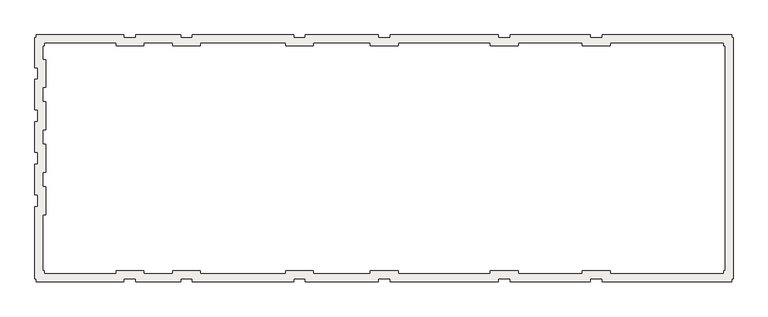
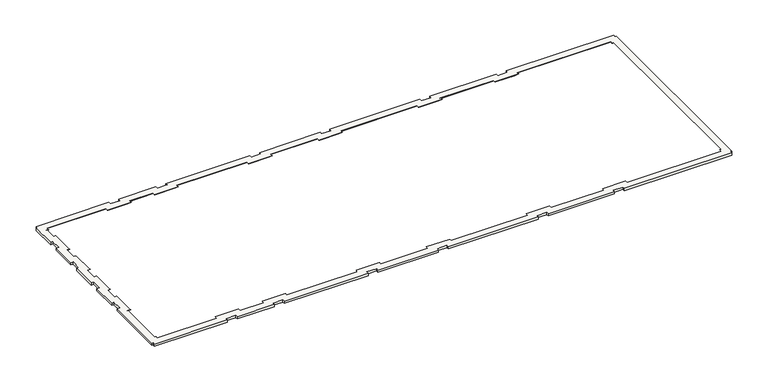
"""IFC4 building model written with IfcOpenShell, lengths in millimetres: slab geometry, HAUNCH FOR SOG : FTS801_Haunch_GS."""

from ifc_helpers import new_model, si_unit, origin, place, context, project, spatial, faceted_brep, source, transform, mapped, element, save


def slab_ae3d626d(model_context):
    return source(origin(), model_context, "Body", "Brep", [
        faceted_brep([(370.0, 38729.5208589, 399.9720055), (370.0, 38729.5208589, 199.9720055), (370.0, 38529.5208589, 199.9720055), (370.0, 38529.5208589, 399.9720055), (770.0, 38329.5208589, 199.9720055), (970.0, 38129.5208589, 399.9720055), (970.0, 37929.5208589, 399.9720055), (770.0, 38129.5208589, 199.9720055), (270.0, 38529.5208589, 199.9720055), (270.0, 38529.5208589, 399.9720055), (870.0, 37929.5208589, 399.9720055), (670.0, 38129.5208589, 199.9720055), (270.0, 36419.5208589, 199.9720055), (270.0, 36419.5208589, 399.9720055), (870.0, 37019.5208589, 399.9720055), (670.0, 36819.5208589, 199.9720055), (470.0, 36419.5208589, 199.9720055), (470.0, 36419.5208589, 399.9720055), (405.0, 36419.5208589, 399.9720055), (1070.0, 37019.5208589, 399.9720055), (870.0, 36819.5208589, 199.9720055), (470.0, 35579.5208589, 199.9720055), (470.0, 35579.5208589, 399.9720055), (1070.0, 34979.5208589, 399.9720055), (870.0, 35179.5208589, 199.9720055), (270.0, 35579.5208589, 199.9720055), (270.0, 35579.5208589, 399.9720055), (405.0, 35579.5208589, 399.9720055), (870.0, 34979.5208589, 399.9720055), (670.0, 35179.5208589, 199.9720055), (270.0, 33419.5208589, 199.9720055), (270.0, 33419.5208589, 399.9720055), (870.0, 34019.5208589, 399.9720055), (670.0, 33819.5208589, 199.9720055), (470.0, 33419.5208589, 199.9720055), (470.0, 33419.5208589, 399.9720055), (405.0, 33419.5208589, 399.9720055), (1070.0, 34019.5208589, 399.9720055), (870.0, 33819.5208589, 199.9720055), (470.0, 32579.5208589, 199.9720055), (470.0, 32579.5208589, 399.9720055), (1070.0, 31979.5208589, 399.9720055), (870.0, 32179.5208589, 199.9720055), (270.0, 32579.5208589, 199.9720055), (270.0, 32579.5208589, 399.9720055), (405.0, 32579.5208589, 399.9720055), (870.0, 31979.5208589, 399.9720055), (670.0, 32179.5208589, 199.9720055), (270.0, 30419.5208589, 199.9720055), (270.0, 30419.5208589, 399.9720055), (870.0, 31019.5208589, 399.9720055), (670.0, 30819.5208589, 199.9720055), (470.0, 30419.5208589, 199.9720055), (470.0, 30419.5208589, 399.9720055), (405.0, 30419.5208589, 399.9720055), (1070.0, 31019.5208589, 399.9720055), (870.0, 30819.5208589, 199.9720055), (470.0, 29579.5208589, 199.9720055), (470.0, 29579.5208589, 399.9720055), (1070.0, 28979.5208589, 399.9720055), (870.0, 29179.5208589, 199.9720055), (270.0, 29579.5208589, 199.9720055), (270.0, 29579.5208589, 399.9720055), (405.0, 29579.5208589, 399.9720055), (870.0, 28979.5208589, 399.9720055), (670.0, 29179.5208589, 199.9720055), (270.0, 27419.5208589, 199.9720055), (270.0, 27419.5208589, 399.9720055), (870.0, 28019.5208589, 399.9720055), (670.0, 27819.5208589, 199.9720055), (470.0, 27419.5208589, 199.9720055), (470.0, 27419.5208589, 399.9720055), (405.0, 27419.5208589, 399.9720055), (1070.0, 28019.5208589, 399.9720055), (870.0, 27819.5208589, 199.9720055), (470.0, 26579.5208589, 199.9720055), (470.0, 26579.5208589, 399.9720055), (1070.0, 25979.5208589, 399.9720055), (870.0, 26179.5208589, 199.9720055), (270.0, 26579.5208589, 199.9720055), (270.0, 26579.5208589, 399.9720055), (405.0, 26579.5208589, 399.9720055), (870.0, 25979.5208589, 399.9720055), (670.0, 26179.5208589, 199.9720055), (270.0, 21469.5208589, 199.9720055), (270.0, 21469.5208589, 399.9720055), (870.0, 22069.5208589, 399.9720055), (670.0, 21869.5208589, 199.9720055), (370.0, 21469.5208589, 199.9720055), (370.0, 21469.5208589, 399.9720055), (970.0, 22069.5208589, 399.9720055), (770.0, 21869.5208589, 199.9720055), (370.0, 21269.5208589, 199.9720055), (370.0, 21269.5208589, 399.9720055), (970.0, 21869.5208589, 399.9720055), (770.0, 21669.5208589, 199.9720055), (6574.0, 21269.5208589, 199.9720055), (6574.0, 21269.5208589, 399.9720055), (5974.0, 21869.5208589, 399.9720055), (6174.0, 21669.5208589, 199.9720055), (6574.0, 21469.5208589, 199.9720055), (6574.0, 21469.5208589, 399.9720055), (5974.0, 22069.5208589, 399.9720055), (6174.0, 21869.5208589, 199.9720055), (7414.0, 21469.5208589, 199.9720055), (7414.0, 21469.5208589, 399.9720055), (8014.0, 22069.5208589, 399.9720055), (7814.0, 21869.5208589, 199.9720055), (7414.0, 21269.5208589, 199.9720055), (7414.0, 21269.5208589, 399.9720055), (8014.0, 21869.5208589, 399.9720055), (7814.0, 21669.5208589, 199.9720055), (10574.0, 21269.5208589, 199.9720055), (10574.0, 21269.5208589, 399.9720055), (9974.0, 21869.5208589, 399.9720055), (10174.0, 21669.5208589, 199.9720055), (10574.0, 21469.5208589, 199.9720055), (10574.0, 21469.5208589, 399.9720055), (9974.0, 22069.5208589, 399.9720055), (10174.0, 21869.5208589, 199.9720055), (11414.0, 21469.5208589, 199.9720055), (11414.0, 21469.5208589, 399.9720055), (12014.0, 22069.5208589, 399.9720055), (11814.0, 21869.5208589, 199.9720055), (11414.0, 21269.5208589, 199.9720055), (11414.0, 21269.5208589, 399.9720055), (12014.0, 21869.5208589, 399.9720055), (11814.0, 21669.5208589, 199.9720055), (18574.0, 21269.5208589, 199.9720055), (18574.0, 21269.5208589, 399.9720055), (17974.0, 21869.5208589, 399.9720055), (18174.0, 21669.5208589, 199.9720055), (18574.0, 21469.5208589, 199.9720055), (18574.0, 21469.5208589, 399.9720055), (17974.0, 22069.5208589, 399.9720055), (18174.0, 21869.5208589, 199.9720055), (19414.0, 21469.5208589, 199.9720055), (19414.0, 21469.5208589, 399.9720055), (20014.0, 22069.5208589, 399.9720055), (19814.0, 21869.5208589, 199.9720055), (19414.0, 21269.5208589, 199.9720055), (19414.0, 21269.5208589, 399.9720055), (20014.0, 21869.5208589, 399.9720055), (19814.0, 21669.5208589, 199.9720055), (24574.0, 21269.5208589, 199.9720055), (24574.0, 21269.5208589, 399.9720055), (23974.0, 21869.5208589, 399.9720055), (24174.0, 21669.5208589, 199.9720055), (24574.0, 21469.5208589, 199.9720055), (24574.0, 21469.5208589, 399.9720055), (23974.0, 22069.5208589, 399.9720055), (24174.0, 21869.5208589, 199.9720055), (25414.0, 21469.5208589, 199.9720055), (25414.0, 21469.5208589, 399.9720055), (26014.0, 22069.5208589, 399.9720055), (25814.0, 21869.5208589, 199.9720055), (25414.0, 21269.5208589, 199.9720055), (25414.0, 21269.5208589, 399.9720055), (26014.0, 21869.5208589, 399.9720055), (25814.0, 21669.5208589, 199.9720055), (33074.0, 21269.5208589, 199.9720055), (33074.0, 21269.5208589, 399.9720055), (32474.0, 21869.5208589, 399.9720055), (32674.0, 21669.5208589, 199.9720055), (33074.0, 21469.5208589, 199.9720055), (33074.0, 21469.5208589, 399.9720055), (32474.0, 22069.5208589, 399.9720055), (32674.0, 21869.5208589, 199.9720055), (33914.0, 21469.5208589, 199.9720055), (33914.0, 21469.5208589, 399.9720055), (34514.0, 22069.5208589, 399.9720055), (34314.0, 21869.5208589, 199.9720055), (33914.0, 21269.5208589, 199.9720055), (33914.0, 21269.5208589, 399.9720055), (34514.0, 21869.5208589, 399.9720055), (34314.0, 21669.5208589, 199.9720055), (39574.0, 21269.5208589, 199.9720055), (39574.0, 21269.5208589, 399.9720055), (38974.0, 21869.5208589, 399.9720055), (39174.0, 21669.5208589, 199.9720055), (39574.0, 21469.5208589, 199.9720055), (39574.0, 21469.5208589, 399.9720055), (38974.0, 22069.5208589, 399.9720055), (39174.0, 21869.5208589, 199.9720055), (40414.0, 21469.5208589, 199.9720055), (40414.0, 21469.5208589, 399.9720055), (41014.0, 22069.5208589, 399.9720055), (40814.0, 21869.5208589, 199.9720055), (40414.0, 21269.5208589, 199.9720055), (40414.0, 21269.5208589, 399.9720055), (41014.0, 21869.5208589, 399.9720055), (40814.0, 21669.5208589, 199.9720055), (49580.0, 21269.5208589, 199.9720055), (49580.0, 21269.5208589, 399.9720055), (48980.0, 21869.5208589, 399.9720055), (49180.0, 21669.5208589, 199.9720055), (49580.0, 21469.5208589, 199.9720055), (49580.0, 21469.5208589, 399.9720055), (48980.0, 22069.5208589, 399.9720055), (49180.0, 21869.5208589, 199.9720055), (49680.0, 21469.5208589, 199.9720055), (49680.0, 21469.5208589, 399.9720055), (49595.0, 21469.5208589, 399.9720055), (49080.0, 22069.5208589, 399.9720055), (49280.0, 21869.5208589, 199.9720055), (49680.0, 38529.5208589, 199.9720055), (49680.0, 38529.5208589, 399.9720055), (49080.0, 37929.5208589, 399.9720055), (49280.0, 38129.5208589, 199.9720055), (49580.0, 38529.5208589, 199.9720055), (49580.0, 38529.5208589, 399.9720055), (49595.0, 38529.5208589, 399.9720055), (48980.0, 37929.5208589, 399.9720055), (49180.0, 38129.5208589, 199.9720055), (49580.0, 38729.5208589, 199.9720055), (49580.0, 38729.5208589, 399.9720055), (48980.0, 38129.5208589, 399.9720055), (49180.0, 38329.5208589, 199.9720055), (40414.0, 38729.5208589, 199.9720055), (40414.0, 38729.5208589, 399.9720055), (41014.0, 38129.5208589, 399.9720055), (40814.0, 38329.5208589, 199.9720055), (40414.0, 38529.5208589, 199.9720055), (40414.0, 38529.5208589, 399.9720055), (41014.0, 37929.5208589, 399.9720055), (40814.0, 38129.5208589, 199.9720055), (39574.0, 38529.5208589, 199.9720055), (39574.0, 38529.5208589, 399.9720055), (38974.0, 37929.5208589, 399.9720055), (39174.0, 38129.5208589, 199.9720055), (39574.0, 38729.5208589, 199.9720055), (39574.0, 38729.5208589, 399.9720055), (38974.0, 38129.5208589, 399.9720055), (39174.0, 38329.5208589, 199.9720055), (33914.0, 38729.5208589, 199.9720055), (33914.0, 38729.5208589, 399.9720055), (34514.0, 38129.5208589, 399.9720055), (34314.0, 38329.5208589, 199.9720055), (33914.0, 38529.5208589, 199.9720055), (33914.0, 38529.5208589, 399.9720055), (34514.0, 37929.5208589, 399.9720055), (34314.0, 38129.5208589, 199.9720055), (33074.0, 38529.5208589, 199.9720055), (33074.0, 38529.5208589, 399.9720055), (32474.0, 37929.5208589, 399.9720055), (32674.0, 38129.5208589, 199.9720055), (33074.0, 38729.5208589, 199.9720055), (33074.0, 38729.5208589, 399.9720055), (32474.0, 38129.5208589, 399.9720055), (32674.0, 38329.5208589, 199.9720055), (25414.0, 38729.5208589, 199.9720055), (25414.0, 38729.5208589, 399.9720055), (26014.0, 38129.5208589, 399.9720055), (25814.0, 38329.5208589, 199.9720055), (25414.0, 38529.5208589, 199.9720055), (25414.0, 38529.5208589, 399.9720055), (26014.0, 37929.5208589, 399.9720055), (25814.0, 38129.5208589, 199.9720055), (24574.0, 38529.5208589, 199.9720055), (24574.0, 38529.5208589, 399.9720055), (23974.0, 37929.5208589, 399.9720055), (24174.0, 38129.5208589, 199.9720055), (24574.0, 38729.5208589, 199.9720055), (24574.0, 38729.5208589, 399.9720055), (23974.0, 38129.5208589, 399.9720055), (24174.0, 38329.5208589, 199.9720055), (19414.0, 38729.5208589, 199.9720055), (19414.0, 38729.5208589, 399.9720055), (20014.0, 38129.5208589, 399.9720055), (19814.0, 38329.5208589, 199.9720055), (19414.0, 38529.5208589, 199.9720055), (19414.0, 38529.5208589, 399.9720055), (20014.0, 37929.5208589, 399.9720055), (19814.0, 38129.5208589, 199.9720055), (18574.0, 38529.5208589, 199.9720055), (18574.0, 38529.5208589, 399.9720055), (17974.0, 37929.5208589, 399.9720055), (18174.0, 38129.5208589, 199.9720055), (18574.0, 38729.5208589, 199.9720055), (18574.0, 38729.5208589, 399.9720055), (17974.0, 38129.5208589, 399.9720055), (18174.0, 38329.5208589, 199.9720055), (11414.0, 38729.5208589, 199.9720055), (11414.0, 38729.5208589, 399.9720055), (12014.0, 38129.5208589, 399.9720055), (11814.0, 38329.5208589, 199.9720055), (11414.0, 38529.5208589, 199.9720055), (11414.0, 38529.5208589, 399.9720055), (12014.0, 37929.5208589, 399.9720055), (11814.0, 38129.5208589, 199.9720055), (10574.0, 38529.5208589, 199.9720055), (10574.0, 38529.5208589, 399.9720055), (9974.0, 37929.5208589, 399.9720055), (10174.0, 38129.5208589, 199.9720055), (10574.0, 38729.5208589, 199.9720055), (10574.0, 38729.5208589, 399.9720055), (9974.0, 38129.5208589, 399.9720055), (10174.0, 38329.5208589, 199.9720055), (7414.0, 38729.5208589, 199.9720055), (7414.0, 38729.5208589, 399.9720055), (8014.0, 38129.5208589, 399.9720055), (7814.0, 38329.5208589, 199.9720055), (7414.0, 38529.5208589, 199.9720055), (7414.0, 38529.5208589, 399.9720055), (8014.0, 37929.5208589, 399.9720055), (7814.0, 38129.5208589, 199.9720055), (6574.0, 38529.5208589, 199.9720055), (6574.0, 38529.5208589, 399.9720055), (5974.0, 37929.5208589, 399.9720055), (6174.0, 38129.5208589, 199.9720055), (6574.0, 38729.5208589, 199.9720055), (6574.0, 38729.5208589, 399.9720055), (5974.0, 38129.5208589, 399.9720055), (6174.0, 38329.5208589, 199.9720055)], [[[0, 1, 2, 3]], [[4, 5, 6, 7]], [[3, 2, 8, 9]], [[7, 6, 10, 11]], [[9, 8, 12, 13]], [[11, 10, 14, 15]], [[13, 12, 16, 17, 18]], [[15, 14, 19, 20]], [[17, 16, 21, 22]], [[20, 19, 23, 24]], [[22, 21, 25, 26, 27]], [[24, 23, 28, 29]], [[26, 25, 30, 31]], [[29, 28, 32, 33]], [[31, 30, 34, 35, 36]], [[33, 32, 37, 38]], [[35, 34, 39, 40]], [[38, 37, 41, 42]], [[40, 39, 43, 44, 45]], [[42, 41, 46, 47]], [[44, 43, 48, 49]], [[47, 46, 50, 51]], [[49, 48, 52, 53, 54]], [[51, 50, 55, 56]], [[53, 52, 57, 58]], [[56, 55, 59, 60]], [[58, 57, 61, 62, 63]], [[60, 59, 64, 65]], [[62, 61, 66, 67]], [[65, 64, 68, 69]], [[67, 66, 70, 71, 72]], [[69, 68, 73, 74]], [[71, 70, 75, 76]], [[74, 73, 77, 78]], [[76, 75, 79, 80, 81]], [[78, 77, 82, 83]], [[80, 79, 84, 85]], [[83, 82, 86, 87]], [[85, 84, 88, 89]], [[87, 86, 90, 91]], [[89, 88, 92, 93]], [[91, 90, 94, 95]], [[93, 92, 96, 97]], [[95, 94, 98, 99]], [[97, 96, 100, 101]], [[99, 98, 102, 103]], [[101, 100, 104, 105]], [[103, 102, 106, 107]], [[105, 104, 108, 109]], [[107, 106, 110, 111]], [[109, 108, 112, 113]], [[111, 110, 114, 115]], [[113, 112, 116, 117]], [[115, 114, 118, 119]], [[117, 116, 120, 121]], [[119, 118, 122, 123]], [[121, 120, 124, 125]], [[123, 122, 126, 127]], [[125, 124, 128, 129]], [[127, 126, 130, 131]], [[129, 128, 132, 133]], [[131, 130, 134, 135]], [[133, 132, 136, 137]], [[135, 134, 138, 139]], [[137, 136, 140, 141]], [[139, 138, 142, 143]], [[141, 140, 144, 145]], [[143, 142, 146, 147]], [[145, 144, 148, 149]], [[147, 146, 150, 151]], [[149, 148, 152, 153]], [[151, 150, 154, 155]], [[153, 152, 156, 157]], [[155, 154, 158, 159]], [[157, 156, 160, 161]], [[159, 158, 162, 163]], [[161, 160, 164, 165]], [[163, 162, 166, 167]], [[165, 164, 168, 169]], [[167, 166, 170, 171]], [[169, 168, 172, 173]], [[171, 170, 174, 175]], [[173, 172, 176, 177]], [[175, 174, 178, 179]], [[177, 176, 180, 181]], [[179, 178, 182, 183]], [[181, 180, 184, 185]], [[183, 182, 186, 187]], [[185, 184, 188, 189]], [[187, 186, 190, 191]], [[189, 188, 192, 193]], [[191, 190, 194, 195]], [[193, 192, 196, 197]], [[195, 194, 198, 199]], [[197, 196, 200, 201, 202]], [[199, 198, 203, 204]], [[201, 200, 205, 206]], [[204, 203, 207, 208]], [[206, 205, 209, 210, 211]], [[208, 207, 212, 213]], [[210, 209, 214, 215]], [[213, 212, 216, 217]], [[215, 214, 218, 219]], [[217, 216, 220, 221]], [[219, 218, 222, 223]], [[221, 220, 224, 225]], [[223, 222, 226, 227]], [[225, 224, 228, 229]], [[227, 226, 230, 231]], [[229, 228, 232, 233]], [[231, 230, 234, 235]], [[233, 232, 236, 237]], [[235, 234, 238, 239]], [[237, 236, 240, 241]], [[239, 238, 242, 243]], [[241, 240, 244, 245]], [[243, 242, 246, 247]], [[245, 244, 248, 249]], [[247, 246, 250, 251]], [[249, 248, 252, 253]], [[251, 250, 254, 255]], [[253, 252, 256, 257]], [[255, 254, 258, 259]], [[257, 256, 260, 261]], [[259, 258, 262, 263]], [[261, 260, 264, 265]], [[263, 262, 266, 267]], [[265, 264, 268, 269]], [[267, 266, 270, 271]], [[269, 268, 272, 273]], [[271, 270, 274, 275]], [[273, 272, 276, 277]], [[275, 274, 278, 279]], [[277, 276, 280, 281]], [[279, 278, 282, 283]], [[281, 280, 284, 285]], [[283, 282, 286, 287]], [[285, 284, 288, 289]], [[287, 286, 290, 291]], [[289, 288, 292, 293]], [[291, 290, 294, 295]], [[293, 292, 296, 297]], [[295, 294, 298, 299]], [[297, 296, 300, 301]], [[299, 298, 302, 303]], [[301, 300, 304, 305]], [[303, 302, 306, 307]], [[305, 304, 308, 309]], [[307, 306, 310, 311]], [[309, 308, 312, 313]], [[311, 310, 1, 0]], [[303, 307, 311, 0, 3, 9, 13, 18, 17, 22, 27, 26, 31, 36, 35, 40, 45, 44, 49, 54, 53, 58, 63, 62, 67, 72, 71, 76, 81, 80, 85, 89, 93, 97, 101, 105, 109, 113, 117, 121, 125, 129, 133, 137, 141, 145, 149, 153, 157, 161, 165, 169, 173, 177, 181, 185, 189, 193, 197, 202, 201, 206, 211, 210, 215, 219, 223, 227, 231, 235, 239, 243, 247, 251, 255, 259, 263, 267, 271, 275, 279, 283, 287, 291, 295, 299], [5, 312, 308, 304, 300, 296, 292, 288, 284, 280, 276, 272, 268, 264, 260, 256, 252, 248, 244, 240, 236, 232, 228, 224, 220, 216, 212, 207, 203, 198, 194, 190, 186, 182, 178, 174, 170, 166, 162, 158, 154, 150, 146, 142, 138, 134, 130, 126, 122, 118, 114, 110, 106, 102, 98, 94, 90, 86, 82, 77, 73, 68, 64, 59, 55, 50, 46, 41, 37, 32, 28, 23, 19, 14, 10, 6]], [[313, 312, 5, 4]], [[1, 310, 306, 302, 298, 294, 290, 286, 282, 278, 274, 270, 266, 262, 258, 254, 250, 246, 242, 238, 234, 230, 226, 222, 218, 214, 209, 205, 200, 196, 192, 188, 184, 180, 176, 172, 168, 164, 160, 156, 152, 148, 144, 140, 136, 132, 128, 124, 120, 116, 112, 108, 104, 100, 96, 92, 88, 84, 79, 75, 70, 66, 61, 57, 52, 48, 43, 39, 34, 30, 25, 21, 16, 12, 8, 2], [305, 309, 313, 4, 7, 11, 15, 20, 24, 29, 33, 38, 42, 47, 51, 56, 60, 65, 69, 74, 78, 83, 87, 91, 95, 99, 103, 107, 111, 115, 119, 123, 127, 131, 135, 139, 143, 147, 151, 155, 159, 163, 167, 171, 175, 179, 183, 187, 191, 195, 199, 204, 208, 213, 217, 221, 225, 229, 233, 237, 241, 245, 249, 253, 257, 261, 265, 269, 273, 277, 281, 285, 289, 293, 297, 301]]]),
    ])


if __name__ == "__main__":
    model = new_model("IFC4")
    model_context = context("Model", 3, world=origin())
    ifc_project = project(units=[si_unit("LENGTHUNIT", "METRE", prefix="MILLI")], contexts=[model_context])
    site = spatial("IfcSite", under=ifc_project)
    building = spatial("IfcBuilding", under=site)
    placement = place(None, origin())
    slab_shape = slab_ae3d626d(model_context)
    element("IfcSlab", 1, ObjectType="HAUNCH FOR SOG : FTS801_Haunch_GS", at=placement, inside=building, context=model_context, shape_type="MappedRepresentation", body=[
        mapped(slab_shape, transform((0.0, 0.0, 0.0), x_axis=(1.0, 0.0, 0.0), y_axis=(0.0, 1.0, 0.0), z_axis=(0.0, 0.0, 1.0))),
    ])
    save(model, "model.ifc")

# Revit data of these elements
# Element 1 (IfcSlab, "HAUNCH FOR SOG : FTS801_Haunch_GS")
#   Materials on its faces: "A03AD032-00010_Structural Concrete_UG_20-24MPa"
# Materials
#   "A03AD032-00010_Structural Concrete_UG_20-24MPa": class "Concrete", colour RGB 176 176 176, transparency 0, Keynote = "09910.A1", Description = "Substructure Concrete / Cement Type-1 / 24MPa", Cost = 0
